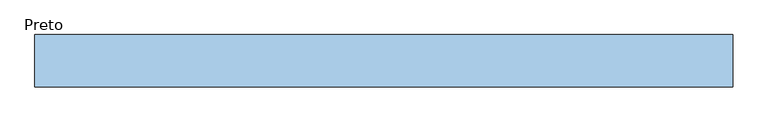
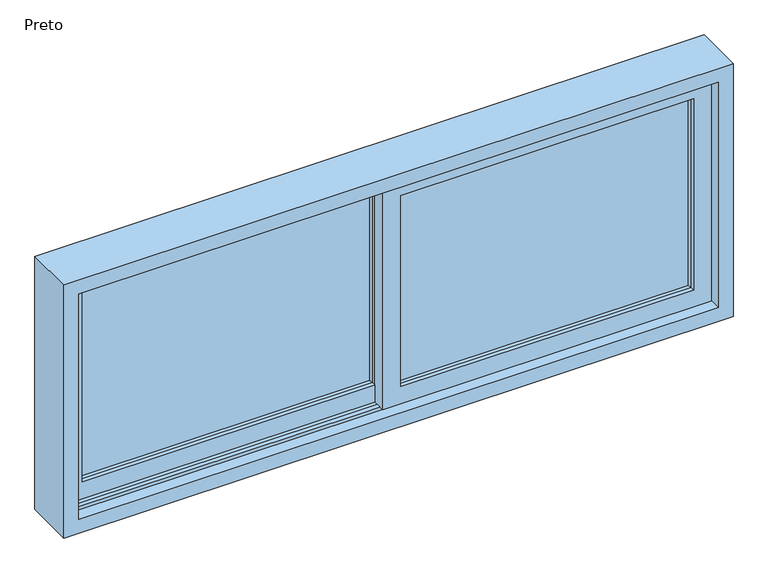
"""IFC4 building model written with IfcOpenShell, lengths in millimetres: window geometry, Blks_Cons Weiku_Janela de Correr 02 Folhas : Preto."""

from ifc_helpers import new_model, si_unit, frame, origin, place, context, project, spatial, polyline, outline, extrude, faceted_brep, source, transform, mapped, element, save


def preto_78440e2c(model_context):
    return source(origin(), model_context, "Body", "SolidModel", [
        faceted_brep([(27.0, -13.0, 898.0), (27.0, -18.0, 898.0), (27.0, -18.0, 1502.0), (27.0, -13.0, 1502.0), (32.0, -18.0, 903.0), (32.0, -18.0, 1497.0), (902.0, -18.0, 1502.0), (902.0, -13.0, 1502.0), (897.0, -18.0, 1497.0), (902.0, -18.0, 898.0), (902.0, -13.0, 898.0), (897.0, -18.0, 903.0)], [[[0, 1, 2, 3]], [[4, 0, 3, 5]], [[3, 2, 6, 7]], [[5, 3, 7, 8]], [[7, 6, 9, 10]], [[8, 7, 10, 11]], [[1, 9, 6, 2], [5, 8, 11, 4]], [[10, 9, 1, 0]], [[11, 10, 0, 4]]]),
        faceted_brep([(902.0, -27.0, 898.0), (902.0, -22.0, 898.0), (902.0, -22.0, 1502.0), (902.0, -27.0, 1502.0), (27.0, -22.0, 1502.0), (27.0, -27.0, 1502.0), (27.0, -22.0, 898.0), (27.0, -27.0, 898.0), (897.0, -22.0, 1497.0), (32.0, -22.0, 1497.0), (32.0, -22.0, 903.0), (897.0, -22.0, 903.0)], [[[0, 1, 2, 3]], [[3, 2, 4, 5]], [[5, 4, 6, 7]], [[1, 6, 4, 2], [8, 9, 10, 11]], [[7, 6, 1, 0]], [[11, 0, 3, 8]], [[8, 3, 5, 9]], [[9, 5, 7, 10]], [[10, 7, 0, 11]]]),
        extrude(outline(polyline([(902.0, -22.0), (27.0, -22.0), (27.0, -18.0), (902.0, -18.0), (902.0, -22.0)])), frame((0.0, 0.0, 898.0), z_axis=(0.0, 0.0, 1.0), x_axis=(1.0, 0.0, 0.0)), (0.0, 0.0, 1.0), 604.0),
        extrude(outline(polyline([(844.0, 956.0), (1556.0, 956.0), (1556.0, -27.0), (844.0, -27.0), (844.0, 956.0)]), holes=[polyline([(1502.0, 27.0), (1502.0, 902.0), (898.0, 902.0), (898.0, 27.0), (1502.0, 27.0)])]), frame((0.0, -40.0, 0.0), z_axis=(0.0, 1.0, 0.0), x_axis=(0.0, 0.0, 1.0)), (0.0, 0.0, 1.0), 40.0),
        faceted_brep([(-902.0, 27.0, 898.0), (-902.0, 22.0, 898.0), (-902.0, 22.0, 1502.0), (-902.0, 27.0, 1502.0), (-897.0, 22.0, 903.0), (-897.0, 22.0, 1497.0), (-27.0, 22.0, 1502.0), (-27.0, 27.0, 1502.0), (-32.0, 22.0, 1497.0), (-27.0, 22.0, 898.0), (-27.0, 27.0, 898.0), (-32.0, 22.0, 903.0)], [[[0, 1, 2, 3]], [[4, 0, 3, 5]], [[3, 2, 6, 7]], [[5, 3, 7, 8]], [[7, 6, 9, 10]], [[8, 7, 10, 11]], [[1, 9, 6, 2], [5, 8, 11, 4]], [[10, 9, 1, 0]], [[11, 10, 0, 4]]]),
        faceted_brep([(-27.0, 13.0, 898.0), (-27.0, 18.0, 898.0), (-27.0, 18.0, 1502.0), (-27.0, 13.0, 1502.0), (-902.0, 18.0, 1502.0), (-902.0, 13.0, 1502.0), (-902.0, 18.0, 898.0), (-902.0, 13.0, 898.0), (-32.0, 18.0, 1497.0), (-897.0, 18.0, 1497.0), (-897.0, 18.0, 903.0), (-32.0, 18.0, 903.0)], [[[0, 1, 2, 3]], [[3, 2, 4, 5]], [[5, 4, 6, 7]], [[1, 6, 4, 2], [8, 9, 10, 11]], [[7, 6, 1, 0]], [[11, 0, 3, 8]], [[8, 3, 5, 9]], [[9, 5, 7, 10]], [[10, 7, 0, 11]]]),
        extrude(outline(polyline([(-27.0, 18.0), (-902.0, 18.0), (-902.0, 22.0), (-27.0, 22.0), (-27.0, 18.0)])), frame((0.0, 0.0, 898.0), z_axis=(0.0, 0.0, 1.0), x_axis=(1.0, 0.0, 0.0)), (0.0, 0.0, 1.0), 604.0),
        extrude(outline(polyline([(844.0, 27.0), (1556.0, 27.0), (1556.0, -956.0), (844.0, -956.0), (844.0, 27.0)]), holes=[polyline([(1502.0, -902.0), (1502.0, -27.0), (898.0, -27.0), (898.0, -902.0), (1502.0, -902.0)])]), frame((0.0, 0.0, 0.0), z_axis=(0.0, 1.0, 0.0), x_axis=(0.0, 0.0, 1.0)), (0.0, 0.0, 1.0), 40.0),
        faceted_brep([(956.0, 75.0, 844.0), (-956.0, 75.0, 844.0), (-956.0, 40.0, 844.0), (956.0, 40.0, 844.0), (-956.0, -75.0, 844.0), (956.0, -75.0, 844.0), (956.0, -40.0, 844.0), (-956.0, -40.0, 844.0), (-956.0, -13.0, 844.0), (-956.0, -27.0, 844.0), (956.0, -27.0, 844.0), (956.0, -13.0, 844.0), (-956.0, 27.0, 844.0), (-956.0, 13.0, 844.0), (956.0, 13.0, 844.0), (956.0, 27.0, 844.0), (1000.0, 75.0, 800.0), (-1000.0, 75.0, 800.0), (-1000.0, 75.0, 1600.0), (1000.0, 75.0, 1600.0), (956.0, 75.0, 1556.0), (-956.0, 75.0, 1556.0), (-956.0, 40.0, 1556.0), (-956.0, 40.0, 1566.0), (-956.0, 27.0, 1566.0), (-956.0, 27.0, 1556.0), (-956.0, 13.0, 1556.0), (-956.0, 13.0, 1566.0), (-956.0, -13.0, 1566.0), (-956.0, -13.0, 1556.0), (-956.0, -27.0, 1556.0), (-956.0, -27.0, 1566.0), (-956.0, -40.0, 1566.0), (-956.0, -40.0, 1556.0), (-956.0, -75.0, 1556.0), (-956.0, -40.0, 834.0), (-956.0, -27.0, 834.0), (-956.0, -13.0, 834.0), (-956.0, 13.0, 834.0), (-956.0, 27.0, 834.0), (-956.0, 40.0, 834.0), (956.0, 40.0, 834.0), (956.0, 27.0, 834.0), (956.0, 13.0, 834.0), (956.0, -13.0, 834.0), (956.0, -27.0, 834.0), (956.0, -40.0, 834.0), (956.0, -75.0, 1556.0), (956.0, -40.0, 1556.0), (956.0, -40.0, 1566.0), (956.0, -27.0, 1566.0), (956.0, -27.0, 1556.0), (956.0, -13.0, 1556.0), (956.0, -13.0, 1566.0), (956.0, 13.0, 1566.0), (956.0, 13.0, 1556.0), (956.0, 27.0, 1556.0), (956.0, 27.0, 1566.0), (956.0, 40.0, 1566.0), (956.0, 40.0, 1556.0), (-1000.0, -75.0, 800.0), (1000.0, -75.0, 800.0), (1000.0, -75.0, 1600.0), (-1000.0, -75.0, 1600.0)], [[[0, 1, 2, 3]], [[4, 5, 6, 7]], [[8, 9, 10, 11]], [[12, 13, 14, 15]], [[16, 17, 18, 19], [1, 0, 20, 21]], [[1, 21, 22, 23, 24, 25, 26, 27, 28, 29, 30, 31, 32, 33, 34, 4, 7, 35, 36, 9, 8, 37, 38, 13, 12, 39, 40, 2]], [[40, 41, 3, 2]], [[20, 0, 3, 41, 42, 15, 14, 43, 44, 11, 10, 45, 46, 6, 5, 47, 48, 49, 50, 51, 52, 53, 54, 55, 56, 57, 58, 59]], [[60, 61, 62, 63], [5, 4, 34, 47]], [[46, 35, 7, 6]], [[45, 10, 9, 36]], [[11, 44, 37, 8]], [[43, 14, 13, 38]], [[15, 42, 39, 12]], [[61, 16, 19, 62]], [[16, 61, 60, 17]], [[17, 60, 63, 18]], [[46, 45, 36, 35]], [[44, 43, 38, 37]], [[42, 41, 40, 39]], [[26, 25, 56, 55]], [[30, 29, 52, 51]], [[21, 20, 59, 22]], [[47, 34, 33, 48]], [[18, 63, 62, 19]], [[55, 54, 27, 26]], [[54, 53, 28, 27]], [[53, 52, 29, 28]], [[51, 50, 31, 30]], [[50, 49, 32, 31]], [[32, 49, 48, 33]], [[58, 23, 22, 59]], [[58, 57, 24, 23]], [[57, 56, 25, 24]]]),
    ])


if __name__ == "__main__":
    model = new_model("IFC4")
    model_context = context("Model", 3, world=origin())
    ifc_project = project(units=[si_unit("LENGTHUNIT", "METRE", prefix="MILLI")], contexts=[model_context])
    site = spatial("IfcSite", under=ifc_project)
    building = spatial("IfcBuilding", under=site)
    placement = place(None, origin())
    preto_shape = preto_78440e2c(model_context)
    element("IfcWindow", 1, ObjectType="Blks_Cons Weiku_Janela de Correr 02 Folhas : Preto", at=placement, inside=building, context=model_context, shape_type="MappedRepresentation", body=[
        mapped(preto_shape, transform((0.0, 0.0, 0.0), x_axis=(1.0, 0.0, 0.0), y_axis=(0.0, 1.0, 0.0), z_axis=(0.0, 0.0, 1.0))),
    ])
    save(model, "model.ifc")

# Revit data of these elements
# Type "Blks_Cons Weiku_Janela de Correr 02 Folhas : Preto"
#   Type Mark = "J26"
#   Type Comments = "Janela de Correr 02 Folhas"
#   Manufacturer = "Weiku"
#   Created By / Criado Por / Creado por = "Blocks"
#   Author URL = "https://BlocksRvt.com/"
#   Author Contact = "info@blocksrvt.com"
#   Assembly Code = "Cons"
#   c [instance default] = 250 mm
#   b [instance default] = 912 mm
#   a [instance default] = 983 mm
#   Rough Width [instance default] = 2000 mm
#   Width [instance default] = 1912 mm
#   Espessura Folha [instance default] = 40 mm
#   Rough Height [instance default] = 1000 mm
#   Height [instance default] = 912 mm
#   Abertura Janela Equerda [instance default] = 0 mm
#   Abertura Janela Direita [instance default] = 0 mm
#   Vidro = .vidro_growarq
#   Vedação = Blks - Rubber - Black
#   Janela = Blks - Plastic - Black - Glazed
#   Wall Closure = (empty or 0)
# Element 1 (IfcWindow, "Blks_Cons Weiku_Janela de Correr 02 Folhas : Preto")
#   c = 200 mm
#   b = 712 mm
#   Rough Height = 800 mm
#   Height = 712 mm
#   Materials on its faces: "Blks - Plastic - Black - Glazed", "Blks - Rubber - Black", ".vidro_growarq"
# Materials
#   ".vidro_growarq": class "Vidro", colour RGB 200 215 215, transparency 0.6, Description = "Vidroverde", Cost = 0
#   "Blks - Rubber - Black": class "Paint/Coating", colour RGB 38 38 38, transparency 0, Cost = 0
#   "Blks - Plastic - Black - Glazed": class "Plastic", colour RGB 25 25 25, transparency 0, Cost = 0
